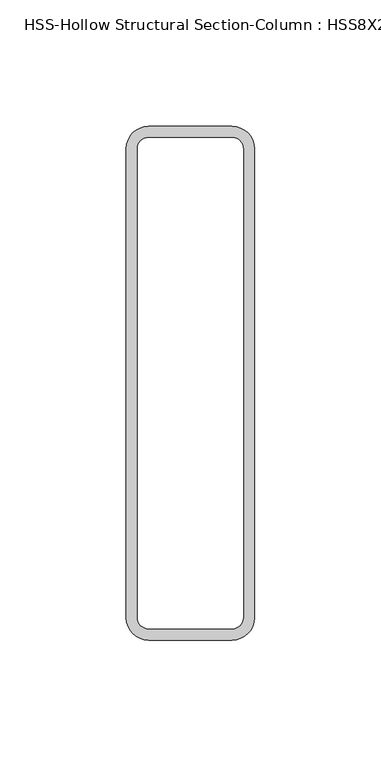
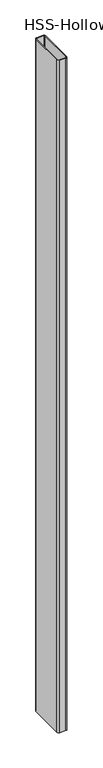
"""IFC4 building model written with IfcOpenShell, lengths in millimetres: column geometry, HSS-Hollow Structural Section-Column : HSS8X2X3/16."""

from ifc_helpers import new_model, si_unit, point, frame, frame_2d, origin, place, context, project, spatial, polyline, circle_curve, trimmed, segment, composite_curve, outline, extrude, source, transform, mapped, element, save


def hss_hollow_structural_section_column_hss8x2x3_16_47370f60(model_context):
    return source(origin(), model_context, "Body", "SweptSolid", [
        extrude(outline(composite_curve([segment(trimmed(circle_curve(frame_2d((16.5608, 92.7608)), 8.8392), [point((16.5608, 101.6))], [point((25.4, 92.7608))], False, "CARTESIAN"), True, "CONTINUOUS"), segment(polyline([(25.4, 92.7608), (25.4, -92.7608)]), True, "CONTINUOUS"), segment(trimmed(circle_curve(frame_2d((16.5608, -92.7608)), 8.8392), [point((25.4, -92.7608))], [point((16.5608, -101.6))], False, "CARTESIAN"), True, "CONTINUOUS"), segment(polyline([(16.5608, -101.6), (-16.5608, -101.6)]), True, "CONTINUOUS"), segment(trimmed(circle_curve(frame_2d((-16.5608, -92.7608)), 8.8392), [point((-16.5608, -101.6))], [point((-25.4, -92.7608))], False, "CARTESIAN"), True, "CONTINUOUS"), segment(polyline([(-25.4, -92.7608), (-25.4, 92.7608)]), True, "CONTINUOUS"), segment(trimmed(circle_curve(frame_2d((-16.5608, 92.7608)), 8.8392), [point((-25.4, 92.7608))], [point((-16.5608, 101.6))], False, "CARTESIAN"), True, "CONTINUOUS"), segment(polyline([(-16.5608, 101.6), (16.5608, 101.6)]), True, "CONTINUOUS")], self_intersect=False), holes=[composite_curve([segment(polyline([(16.5608, 97.1804), (-16.5608, 97.1804)]), True, "CONTINUOUS"), segment(trimmed(circle_curve(frame_2d((-16.5608, 92.7608)), 4.4196), [point((-16.5608, 97.1804))], [point((-20.9804, 92.7608))], True, "CARTESIAN"), True, "CONTINUOUS"), segment(polyline([(-20.9804, 92.7608), (-20.9804, -92.7608)]), True, "CONTINUOUS"), segment(trimmed(circle_curve(frame_2d((-16.5608, -92.7608)), 4.4196), [point((-20.9804, -92.7608))], [point((-16.5608, -97.1804))], True, "CARTESIAN"), True, "CONTINUOUS"), segment(polyline([(-16.5608, -97.1804), (16.5608, -97.1804)]), True, "CONTINUOUS"), segment(trimmed(circle_curve(frame_2d((16.5608, -92.7608)), 4.4196), [point((16.5608, -97.1804))], [point((20.9804, -92.7608))], True, "CARTESIAN"), True, "CONTINUOUS"), segment(polyline([(20.9804, -92.7608), (20.9804, 92.7608)]), True, "CONTINUOUS"), segment(trimmed(circle_curve(frame_2d((16.5608, 92.7608)), 4.4196), [point((20.9804, 92.7608))], [point((16.5608, 97.1804))], True, "CARTESIAN"), True, "CONTINUOUS")], self_intersect=False)]), frame((0.0, 0.0, -1200.0), z_axis=(0.0, 0.0, 1.0), x_axis=(1.0, 0.0, 0.0)), (0.0, 0.0, 1.0), 3644.0),
    ])


if __name__ == "__main__":
    model = new_model("IFC4")
    model_context = context("Model", 3, world=origin())
    ifc_project = project(units=[si_unit("LENGTHUNIT", "METRE", prefix="MILLI")], contexts=[model_context])
    site = spatial("IfcSite", under=ifc_project)
    building = spatial("IfcBuilding", under=site)
    placement = place(None, origin())
    hss_hollow_structural_section_column_hss8x2x3_16_shape = hss_hollow_structural_section_column_hss8x2x3_16_47370f60(model_context)
    element("IfcColumn", 1, ObjectType="HSS-Hollow Structural Section-Column : HSS8X2X3/16", at=placement, inside=building, context=model_context, shape_type="MappedRepresentation", body=[
        mapped(hss_hollow_structural_section_column_hss8x2x3_16_shape, transform((0.0, 0.0, 0.0), x_axis=(1.0, 0.0, 0.0), y_axis=(0.0, 1.0, 0.0), z_axis=(0.0, 0.0, 1.0))),
    ])
    save(model, "model.ifc")

# Revit data of these elements
# Type "HSS-Hollow Structural Section-Column : HSS8X2X3/16"
#   Assembly Code = "B10"
#   Shape = "Rect."
#   Cost = 1
#   W = 12
#   Ht = 203.2 mm
#   b = 50.8 mm
#   kr = 8.839 mm
#   t = 4.42 mm
#   A = 0.00211612 m²
#   Structural Material [instance default] = Steel ASTM A500, Grade B, Rectangular and Square
# Element 1 (IfcColumn, "HSS-Hollow Structural Section-Column : HSS8X2X3/16")
#   Structural Material = Metal - Steel 43-275
#   Materials on its faces: "Metal - Steel 43-275"
# Materials
#   "Steel ASTM A500, Grade B, Rectangular and Square": class "Metal", colour RGB 199 199 199, transparency 0, Description = "Carbon steel", Cost = 0
#   "Metal - Steel 43-275": class "Metal", colour RGB 247 247 247, transparency 0, Cost = 0
